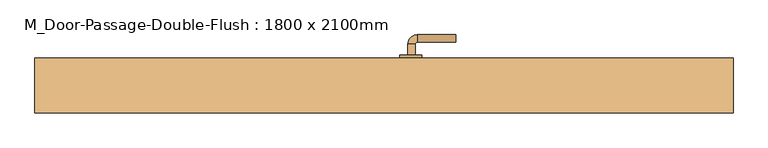
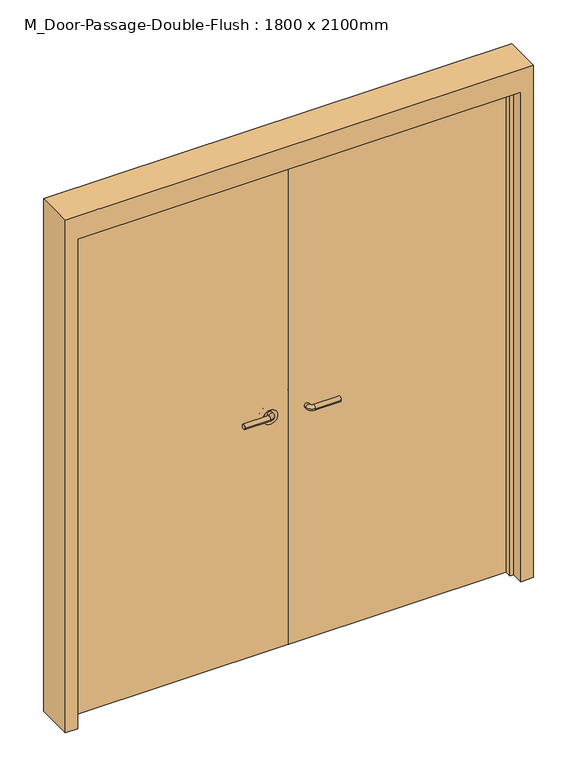
"""IFC4 building model written with IfcOpenShell, lengths in millimetres: door geometry, M_Door-Passage-Double-Flush : 1800 x 2100mm."""

import ifcopenshell
import ifcopenshell.guid

model = None  # the IFC model being written
_history = None  # IfcOwnerHistory: only IFC2X3 demands one
_inside = {}  # id of a spatial element -> (the spatial element, [elements in it])
_under = {}  # id of a project, library or spatial element -> (it, [spatial elements below it])
_declared = {}  # id of a project -> (the project, [libraries it declares])
_typed = {}  # id of a type object -> (the type object, [elements of that type])
_made_of = {}  # id of a material, layer set ... -> (it, [elements and type objects made of it])


def new_model(schema):
    """Start an empty IFC model of exactly this schema.

    Asked for "IFC4X3", IfcOpenShell would pick the latest addendum, in which some entities
    have other attributes; the version numbers below select the first issue.
    IFC2X3 requires an IfcOwnerHistory on every rooted entity: one is made here for all.
    """
    global model, _history
    if schema == "IFC4X3":
        model = ifcopenshell.file(schema_version=(4, 3, 0, 0))
    else:
        model = ifcopenshell.file(schema=schema)
    _inside.clear()
    _under.clear()
    _declared.clear()
    _typed.clear()
    _made_of.clear()
    _history = None
    if model.schema == "IFC2X3":
        org = make("IfcOrganization", Name="unknown")
        user = make(
            "IfcPersonAndOrganization",
            ThePerson=make("IfcPerson", FamilyName="unknown"),
            TheOrganization=org,
        )
        app = make(
            "IfcApplication",
            ApplicationDeveloper=org,
            Version="unknown",
            ApplicationFullName="unknown",
            ApplicationIdentifier="unknown",
        )
        _history = make(
            "IfcOwnerHistory",
            OwningUser=user,
            OwningApplication=app,
            ChangeAction="ADDED",
            CreationDate=0,
        )
    return model


def make(cls, **values):
    """One entity of the class cls with the attributes given. An attribute that is None is left unset."""
    return model.create_entity(
        cls, **{name: value for name, value in values.items() if value is not None}
    )


def rooted(cls, **values):
    """An entity with a GlobalId (a new one), such as an element, a storey or a relation."""
    return make(cls, GlobalId=ifcopenshell.guid.new(), OwnerHistory=_history, **values)


def si_unit(unit_type, name, prefix=None):
    """IfcSIUnit, for example si_unit("LENGTHUNIT", "METRE", prefix="MILLI")."""
    return make("IfcSIUnit", UnitType=unit_type, Prefix=prefix, Name=name)


def assignment(units):
    """IfcUnitAssignment: the units of a project."""
    return None if units is None else make("IfcUnitAssignment", Units=units)


def point(xyz):
    """IfcCartesianPoint."""
    return None if xyz is None else make("IfcCartesianPoint", Coordinates=xyz)


def direction(xyz):
    """IfcDirection."""
    return None if xyz is None else make("IfcDirection", DirectionRatios=xyz)


def frame(location, z_axis=None, x_axis=None):
    """IfcAxis2Placement3D, a coordinate frame: its origin and axes. An axis left out is left unset."""
    return make(
        "IfcAxis2Placement3D",
        Location=point(location),
        Axis=direction(z_axis),
        RefDirection=direction(x_axis),
    )


def frame_2d(location, x_axis=None):
    """IfcAxis2Placement2D, a coordinate frame in the plane: its origin and x axis."""
    return make(
        "IfcAxis2Placement2D", Location=point(location), RefDirection=direction(x_axis)
    )


def origin():
    """The frame at (0, 0, 0) with its axes left unset."""
    return frame((0.0, 0.0, 0.0))


def origin_with_axes():
    """The frame at (0, 0, 0) with the z axis (0, 0, 1) and the x axis (1, 0, 0) written out."""
    return frame((0.0, 0.0, 0.0), z_axis=(0.0, 0.0, 1.0), x_axis=(1.0, 0.0, 0.0))


def place(relative_to, where):
    """IfcLocalPlacement: puts the frame where relative to a parent placement (None: the world)."""
    return make(
        "IfcLocalPlacement", PlacementRelTo=relative_to, RelativePlacement=where
    )


def context(
    kind, dimensions, precision=None, world=None, true_north=None, identifier=None
):
    """IfcGeometricRepresentationContext, for example the 3D "Model" context."""
    return make(
        "IfcGeometricRepresentationContext",
        ContextIdentifier=identifier,
        ContextType=kind,
        CoordinateSpaceDimension=dimensions,
        Precision=precision,
        WorldCoordinateSystem=world,
        TrueNorth=true_north,
    )


def project(units=None, contexts=None):
    """IfcProject with its units and contexts."""
    return rooted(
        "IfcProject",
        Name="project",
        RepresentationContexts=contexts,
        UnitsInContext=assignment(units),
    )


def spatial(cls, under=None, at=None, **own):
    """A site, building, storey or space (cls), placed at a placement, below another one or the project."""
    s = rooted(cls, ObjectPlacement=at, **own)
    if under is not None:
        _under.setdefault(under.id(), (under, []))[1].append(s)
    return s


def polyline(points):
    """IfcPolyline through the points."""
    return make("IfcPolyline", Points=[point(p) for p in points])


def circle_curve(where, radius):
    """IfcCircle in the frame where."""
    return make("IfcCircle", Position=where, Radius=radius)


def ellipse_curve(where, semi_axis1, semi_axis2):
    """IfcEllipse in the frame where."""
    return make(
        "IfcEllipse", Position=where, SemiAxis1=semi_axis1, SemiAxis2=semi_axis2
    )


def trimmed(basis, trim1, trim2, sense, master):
    """IfcTrimmedCurve: the piece of a basis curve between two trims."""
    return make(
        "IfcTrimmedCurve",
        BasisCurve=basis,
        Trim1=trim1,
        Trim2=trim2,
        SenseAgreement=sense,
        MasterRepresentation=master,
    )


def segment(curve, same_sense, transition):
    """IfcCompositeCurveSegment."""
    return make(
        "IfcCompositeCurveSegment",
        Transition=transition,
        SameSense=same_sense,
        ParentCurve=curve,
    )


def composite_curve(segments, self_intersect=None):
    """IfcCompositeCurve: segments joined end to end."""
    return make("IfcCompositeCurve", Segments=segments, SelfIntersect=self_intersect)


def outline(outer, holes=None, kind="AREA"):
    """IfcArbitraryClosedProfileDef: a profile drawn as a closed curve; with holes, ...WithVoids."""
    if holes is None:
        return make("IfcArbitraryClosedProfileDef", ProfileType=kind, OuterCurve=outer)
    return make(
        "IfcArbitraryProfileDefWithVoids",
        ProfileType=kind,
        OuterCurve=outer,
        InnerCurves=holes,
    )


def extrude(swept, where, along, depth):
    """IfcExtrudedAreaSolid: the profile swept, set in the frame where, extruded along a direction by depth."""
    return make(
        "IfcExtrudedAreaSolid",
        SweptArea=swept,
        Position=where,
        ExtrudedDirection=direction(along),
        Depth=depth,
    )


def faces_of(points, faces, orient=None, outer=None):
    """IfcFace entities. A face is a list of loops; a loop is a list of indices into points, from 0.

    orient and outer hold one flag for each loop. By default every Orientation is true, the
    first loop of a face is its IfcFaceOuterBound and the others are IfcFaceBound.
    """
    made = []
    for i, loops in enumerate(faces):
        bounds = []
        for j, loop in enumerate(loops):
            is_outer = j == 0 if outer is None else outer[i][j]
            bounds.append(
                make(
                    "IfcFaceOuterBound" if is_outer else "IfcFaceBound",
                    Bound=make("IfcPolyLoop", Polygon=[points[k] for k in loop]),
                    Orientation=True if orient is None else orient[i][j],
                )
            )
        made.append(make("IfcFace", Bounds=bounds))
    return made


def faceted_brep(points, faces, orient=None, outer=None, voids=None):
    """IfcFacetedBrep: a solid bounded by flat faces; with voids (closed shells), ...WithVoids."""
    shared = [point(p) for p in points]
    hull = make("IfcClosedShell", CfsFaces=faces_of(shared, faces, orient, outer))
    if voids is None:
        return make("IfcFacetedBrep", Outer=hull)
    return make(
        "IfcFacetedBrepWithVoids",
        Outer=hull,
        Voids=[
            make(cls, CfsFaces=faces_of(shared, fs, o, b)) for cls, fs, o, b in voids
        ],
    )


def shape(context_of_items, identifier, shape_type, items):
    """IfcShapeRepresentation: the items that make up one representation, for example the "Body"."""
    return make(
        "IfcShapeRepresentation",
        ContextOfItems=context_of_items,
        RepresentationIdentifier=identifier,
        RepresentationType=shape_type,
        Items=items,
    )


def source(mapping_origin, context_of_items, identifier, shape_type, items):
    """IfcRepresentationMap: a shape defined once, which mapped items show again and again."""
    return make(
        "IfcRepresentationMap",
        MappingOrigin=mapping_origin,
        MappedRepresentation=shape(context_of_items, identifier, shape_type, items),
    )


def transform(
    local_origin,
    x_axis=None,
    y_axis=None,
    z_axis=None,
    scale=None,
    scale2=None,
    scale3=None,
    uniform=True,
):
    """IfcCartesianTransformationOperator3D, or its non-uniform kind. x_axis, y_axis, z_axis: its Axis1, 2, 3."""
    if uniform:
        return make(
            "IfcCartesianTransformationOperator3D",
            Axis1=direction(x_axis),
            Axis2=direction(y_axis),
            LocalOrigin=point(local_origin),
            Scale=scale,
            Axis3=direction(z_axis),
        )
    return make(
        "IfcCartesianTransformationOperator3DnonUniform",
        Axis1=direction(x_axis),
        Axis2=direction(y_axis),
        LocalOrigin=point(local_origin),
        Scale=scale,
        Axis3=direction(z_axis),
        Scale2=scale2,
        Scale3=scale3,
    )


def mapped(mapping_source, mapping_target):
    """IfcMappedItem: shows the shape of a source again, moved by a transform."""
    return make(
        "IfcMappedItem", MappingSource=mapping_source, MappingTarget=mapping_target
    )


def made_of(thing, what):
    """Note that an element or type object is made of a material, layer set ...; save() writes the relation."""
    if what is not None:
        _made_of.setdefault(what.id(), (what, []))[1].append(thing)
    return thing


def element(
    cls,
    number,
    at=None,
    inside=None,
    cuts=None,
    type_object=None,
    material=None,
    context=None,
    identifier="Body",
    shape_type=None,
    held_by="IfcProductDefinitionShape",
    body=None,
    shapes=None,
    **own,
):
    """One element of the class cls, such as IfcWall. Its Tag is "e" and its number.

    at: its placement. inside: the storey or other place that contains it. cuts: it is an
    opening in that element (IfcRelVoidsElement). A single representation is given by context,
    identifier, shape_type and body (its items); several are given by shapes. held_by: the class
    of the entity that holds the representations. save() writes the other relations.
    """
    e = rooted(cls, Tag="e%d" % number, ObjectPlacement=at, **own)
    if body is not None:
        shapes = [shape(context, identifier, shape_type, body)]
    if shapes is not None:
        e.Representation = make(held_by, Representations=shapes)
    if inside is not None:
        _inside.setdefault(inside.id(), (inside, []))[1].append(e)
    if cuts is not None:
        rooted(
            "IfcRelVoidsElement", RelatingBuildingElement=cuts, RelatedOpeningElement=e
        )
    if type_object is not None:
        _typed.setdefault(type_object.id(), (type_object, []))[1].append(e)
    return made_of(e, material)


def aggregate(whole, parts):
    """IfcRelAggregates: a whole, such as a stair, and the parts it consists of."""
    return rooted("IfcRelAggregates", RelatingObject=whole, RelatedObjects=parts)


def save(model, path):
    """Write the relations noted so far, then the file.

    IfcRelAggregates (storeys below a building ...), IfcRelContainedInSpatialStructure (elements
    in a storey), IfcRelDefinesByType, IfcRelAssociatesMaterial and IfcRelDeclares: one each for
    every whole, place, type object, material and project.
    """
    for whole, parts in _under.values():
        aggregate(whole, parts)
    for where, things in _inside.values():
        rooted(
            "IfcRelContainedInSpatialStructure",
            RelatedElements=things,
            RelatingStructure=where,
        )
    for kind, things in _typed.values():
        rooted("IfcRelDefinesByType", RelatedObjects=things, RelatingType=kind)
    for what, things in _made_of.values():
        rooted("IfcRelAssociatesMaterial", RelatedObjects=things, RelatingMaterial=what)
    for by, libraries in _declared.values():
        rooted("IfcRelDeclares", RelatingContext=by, RelatedDefinitions=libraries)
    model.write(path)


def plane_surface(at):
    """IfcPlane: the flat surface through the origin of the frame at, square to its z axis."""
    return make("IfcPlane", Position=at)


def cylinder_surface(at, radius):
    """IfcCylindricalSurface: all points at the distance radius from the z axis of the frame at."""
    return make("IfcCylindricalSurface", Position=at, Radius=radius)


def revolved_surface(curve, axis_point, axis_direction):
    """IfcSurfaceOfRevolution: the curve turned about the line through axis_point along axis_direction."""
    return make(
        "IfcSurfaceOfRevolution",
        SweptCurve=make("IfcArbitraryOpenProfileDef", ProfileType="CURVE", Curve=curve),
        AxisPosition=make("IfcAxis1Placement", Location=point(axis_point), Axis=direction(axis_direction)),
    )


def advanced_brep(points, edges, surfaces, faces):
    """IfcAdvancedBrep: a solid bounded by faces that lie on surfaces and meet in shared edges.

    An edge is (start, end): straight between two places in points (the first is 0);
    or (start, end, curve); or (start, end, curve, False) where it runs against its curve.
    A face is (place in surfaces, loops), or (place, loops, False) where it looks against
    its surface's normal. A loop lists edges by number (the first is 1), with a minus sign
    where the edge is run from its end to its start. The first loop is the outer one.
    """
    corners = [point(p) for p in points]
    vertices = [make("IfcVertexPoint", VertexGeometry=c) for c in corners]
    made = []
    for start, end, *more in edges:
        made.append(
            make(
                "IfcEdgeCurve",
                EdgeStart=vertices[start],
                EdgeEnd=vertices[end],
                EdgeGeometry=more[0] if more else make("IfcPolyline", Points=[corners[start], corners[end]]),
                SameSense=more[1] if len(more) > 1 else True,
            )
        )
    hull = []
    for where, loops, *sense in faces:
        bounds = []
        for j, loop in enumerate(loops):
            ring = [make("IfcOrientedEdge", EdgeElement=made[abs(k) - 1], Orientation=k > 0) for k in loop]
            bounds.append(
                make(
                    "IfcFaceOuterBound" if j == 0 else "IfcFaceBound",
                    Bound=make("IfcEdgeLoop", EdgeList=ring),
                    Orientation=True,
                )
            )
        hull.append(make("IfcAdvancedFace", Bounds=bounds, FaceSurface=surfaces[where], SameSense=sense[0] if sense else True))
    return make("IfcAdvancedBrep", Outer=make("IfcClosedShell", CfsFaces=hull))


def m_door_passage_double_flush_1800_x_2100mm_17443fe2(model_context):
    return source(origin(), model_context, "Body", "SolidModel", [
        advanced_brep(
        [(-65.009375, 102.85, 1016.0), (-85.009375, 102.85, 1016.0), (-65.009375, 72.85, 1016.0), (-85.009375, 72.85, 1016.0), (-90.009375, 67.85, 1016.0), (-90.009375, 47.85, 1016.0), (-195.009375, 47.85, 1016.0), (-195.009375, 67.85, 1016.0)],
        [
            (0, 1, circle_curve(frame((-75.009375, 102.85, 1016.0), z_axis=(0.0, 1.0, 0.0), x_axis=(-1.0, 0.0, 0.0)), 10.0)),
            (1, 0, circle_curve(frame((-75.009375, 102.85, 1016.0), z_axis=(0.0, 1.0, 0.0), x_axis=(-1.0, 0.0, 0.0)), 10.0)),
            (0, 2),
            (2, 3, circle_curve(frame((-75.009375, 72.85, 1016.0), z_axis=(0.0, 1.0, 0.0), x_axis=(-1.0, 0.0, 0.0)), 10.0)),
            (3, 1),
            (3, 2, circle_curve(frame((-75.009375, 72.85, 1016.0), z_axis=(0.0, 1.0, 0.0), x_axis=(-1.0, 0.0, 0.0)), 10.0)),
            (4, 3, circle_curve(frame((-90.009375, 72.85, 1016.0), z_axis=(0.0, 0.0, 1.0), x_axis=(1.0, 0.0, 0.0)), 5.0)),
            (2, 5, circle_curve(frame((-90.009375, 72.85, 1016.0), z_axis=(0.0, 0.0, -1.0), x_axis=(1.0, 0.0, 0.0)), 25.0)),
            (5, 4, circle_curve(frame((-90.009375, 57.85, 1016.0), z_axis=(1.0, 0.0, 0.0), x_axis=(0.0, 1.0, 0.0)), 10.0)),
            (4, 5, circle_curve(frame((-90.009375, 57.85, 1016.0), z_axis=(1.0, 0.0, 0.0), x_axis=(0.0, 1.0, 0.0)), 10.0)),
            (6, 7, circle_curve(frame((-195.009375, 57.85, 1016.0), z_axis=(-1.0, 0.0, 0.0), x_axis=(0.0, 1.0, 0.0)), 10.0)),
            (7, 6, circle_curve(frame((-195.009375, 57.85, 1016.0), z_axis=(-1.0, 0.0, 0.0), x_axis=(0.0, 1.0, 0.0)), 10.0)),
            (5, 6),
            (7, 4),
        ],
        [
            plane_surface(frame((-75.009375, 102.85, 1016.0), z_axis=(0.0, 1.0, 0.0), x_axis=(0.0, 0.0, 1.0))),
            cylinder_surface(frame((-75.009375, 102.85, 1016.0), z_axis=(0.0, 1.0, 0.0), x_axis=(-1.0, 0.0, 0.0)), 10.0),
            revolved_surface(trimmed(ellipse_curve(frame((-75.009375, 72.85, 1016.0), z_axis=(0.0, 1.0, 0.0), x_axis=(-1.0, 0.0, 0.0)), 10.0, 10.0), [point((-65.009375, 72.85, 1016.0))], [point((-85.009375, 72.85, 1016.0))], True, "CARTESIAN"), (-90.009375, 72.85, 1016.0), (0.0, 0.0, -1.0)),
            revolved_surface(trimmed(ellipse_curve(frame((-75.009375, 72.85, 1016.0), z_axis=(0.0, 1.0, 0.0), x_axis=(-1.0, 0.0, 0.0)), 10.0, 10.0), [point((-85.009375, 72.85, 1016.0))], [point((-65.009375, 72.85, 1016.0))], True, "CARTESIAN"), (-90.009375, 72.85, 1016.0), (0.0, 0.0, -1.0)),
            plane_surface(frame((-195.009375, 57.85, 1016.0), z_axis=(-1.0, 0.0, 0.0), x_axis=(0.0, 0.0, 1.0))),
            cylinder_surface(frame((-90.009375, 57.85, 1016.0), z_axis=(1.0, 0.0, 0.0), x_axis=(0.0, 1.0, 0.0)), 10.0),
        ],
        [
            (0, [[1, 2]]),
            (1, [[-1, 3, 4, 5]]),
            (1, [[-2, -5, 6, -3]]),
            (2, [[7, -4, 8, 9]]),
            (3, [[-8, -6, -7, 10]]),
            (4, [[11, 12]]),
            (5, [[-9, 13, -12, 14]]),
            (5, [[-10, -14, -11, -13]]),
        ],
    ),
        extrude(outline(composite_curve([segment(trimmed(circle_curve(frame_2d((1016.0, -72.509375)), 30.0), [point((1016.0, -42.509375))], [point((1016.0, -102.509375))], False, "CARTESIAN"), True, "CONTINUOUS"), segment(trimmed(circle_curve(frame_2d((1016.0, -72.509375)), 30.0), [point((1016.0, -102.509375))], [point((1016.0, -42.509375))], False, "CARTESIAN"), True, "CONTINUOUS")], self_intersect=False)), frame((0.0, 102.85, 0.0), z_axis=(0.0, 1.0, 0.0), x_axis=(0.0, 0.0, 1.0)), (0.0, 0.0, 1.0), 8.0),
        advanced_brep(
        [(-65.009375, 90.95, 1000.0), (-85.009375, 90.95, 1000.0), (-85.009375, 120.95, 1000.0), (-65.009375, 120.95, 1000.0), (-90.009375, 125.95, 1000.0), (-90.009375, 145.95, 1000.0), (-195.009375, 145.95, 1000.0), (-195.009375, 125.95, 1000.0)],
        [
            (0, 1, circle_curve(frame((-75.009375, 90.95, 1000.0), z_axis=(0.0, -1.0, 0.0), x_axis=(-1.0, 0.0, 0.0)), 10.0)),
            (1, 0, circle_curve(frame((-75.009375, 90.95, 1000.0), z_axis=(0.0, -1.0, 0.0), x_axis=(-1.0, 0.0, 0.0)), 10.0)),
            (1, 2),
            (2, 3, circle_curve(frame((-75.009375, 120.95, 1000.0), z_axis=(0.0, -1.0, 0.0), x_axis=(-1.0, 0.0, 0.0)), 10.0)),
            (3, 0),
            (3, 2, circle_curve(frame((-75.009375, 120.95, 1000.0), z_axis=(0.0, -1.0, 0.0), x_axis=(-1.0, 0.0, 0.0)), 10.0)),
            (4, 5, circle_curve(frame((-90.009375, 135.95, 1000.0), z_axis=(1.0, 0.0, 0.0), x_axis=(0.0, -1.0, 0.0)), 10.0)),
            (5, 3, circle_curve(frame((-90.009375, 120.95, 1000.0), z_axis=(0.0, 0.0, -1.0), x_axis=(1.0, 0.0, 0.0)), 25.0)),
            (2, 4, circle_curve(frame((-90.009375, 120.95, 1000.0), z_axis=(0.0, 0.0, 1.0), x_axis=(1.0, 0.0, 0.0)), 5.0)),
            (5, 4, circle_curve(frame((-90.009375, 135.95, 1000.0), z_axis=(1.0, 0.0, 0.0), x_axis=(0.0, -1.0, 0.0)), 10.0)),
            (6, 7, circle_curve(frame((-195.009375, 135.95, 1000.0), z_axis=(-1.0, 0.0, 0.0), x_axis=(0.0, -1.0, 0.0)), 10.0)),
            (7, 6, circle_curve(frame((-195.009375, 135.95, 1000.0), z_axis=(-1.0, 0.0, 0.0), x_axis=(0.0, -1.0, 0.0)), 10.0)),
            (4, 7),
            (6, 5),
        ],
        [
            plane_surface(frame((-75.009375, 90.95, 1000.0), z_axis=(0.0, -1.0, 0.0), x_axis=(0.0, 0.0, 1.0))),
            cylinder_surface(frame((-75.009375, 90.95, 1000.0), z_axis=(0.0, -1.0, 0.0), x_axis=(-1.0, 0.0, 0.0)), 10.0),
            revolved_surface(trimmed(ellipse_curve(frame((-75.009375, 120.95, 1000.0), z_axis=(0.0, 1.0, 0.0), x_axis=(-1.0, 0.0, 0.0)), 10.0, 10.0), [point((-65.009375, 120.95, 1000.0))], [point((-85.009375, 120.95, 1000.0))], True, "CARTESIAN"), (-90.009375, 120.95, 1000.0), (0.0, 0.0, -1.0)),
            revolved_surface(trimmed(ellipse_curve(frame((-75.009375, 120.95, 1000.0), z_axis=(0.0, 1.0, 0.0), x_axis=(-1.0, 0.0, 0.0)), 10.0, 10.0), [point((-85.009375, 120.95, 1000.0))], [point((-65.009375, 120.95, 1000.0))], True, "CARTESIAN"), (-90.009375, 120.95, 1000.0), (0.0, 0.0, -1.0)),
            plane_surface(frame((-195.009375, 135.95, 1000.0), z_axis=(-1.0, 0.0, 0.0), x_axis=(0.0, 0.0, 1.0))),
            cylinder_surface(frame((-90.009375, 135.95, 1000.0), z_axis=(1.0, 0.0, 0.0), x_axis=(0.0, -1.0, 0.0)), 10.0),
        ],
        [
            (0, [[1, 2]]),
            (1, [[3, 4, 5, -2]]),
            (1, [[-5, 6, -3, -1]]),
            (2, [[7, 8, -4, 9]]),
            (3, [[10, -9, -6, -8]]),
            (4, [[11, 12]]),
            (5, [[13, -11, 14, -7]]),
            (5, [[-14, -12, -13, -10]]),
        ],
    ),
        extrude(outline(composite_curve([segment(trimmed(circle_curve(frame_2d((1000.0, -72.509375)), 30.0), [point((1000.0, -42.509375))], [point((1000.0, -102.509375))], False, "CARTESIAN"), True, "CONTINUOUS"), segment(trimmed(circle_curve(frame_2d((1000.0, -72.509375)), 30.0), [point((1000.0, -102.509375))], [point((1000.0, -42.509375))], False, "CARTESIAN"), True, "CONTINUOUS")], self_intersect=False)), frame((0.0, 82.95, 0.0), z_axis=(0.0, 1.0, 0.0), x_axis=(0.0, 0.0, 1.0)), (0.0, 0.0, 1.0), 8.0),
        advanced_brep(
        [(65.009375, 102.85, 1000.0), (85.009375, 102.85, 1000.0), (85.009375, 72.85, 1000.0), (65.009375, 72.85, 1000.0), (90.009375, 67.85, 1000.0), (90.009375, 47.85, 1000.0), (195.009375, 47.85, 1000.0), (195.009375, 67.85, 1000.0)],
        [
            (0, 1, circle_curve(frame((75.009375, 102.85, 1000.0), z_axis=(0.0, 1.0, 0.0), x_axis=(1.0, 0.0, 0.0)), 10.0)),
            (1, 0, circle_curve(frame((75.009375, 102.85, 1000.0), z_axis=(0.0, 1.0, 0.0), x_axis=(1.0, 0.0, 0.0)), 10.0)),
            (1, 2),
            (2, 3, circle_curve(frame((75.009375, 72.85, 1000.0), z_axis=(0.0, 1.0, 0.0), x_axis=(1.0, 0.0, 0.0)), 10.0)),
            (3, 0),
            (3, 2, circle_curve(frame((75.009375, 72.85, 1000.0), z_axis=(0.0, 1.0, 0.0), x_axis=(1.0, 0.0, 0.0)), 10.0)),
            (4, 5, circle_curve(frame((90.009375, 57.85, 1000.0), z_axis=(-1.0, 0.0, 0.0), x_axis=(0.0, 1.0, 0.0)), 10.0)),
            (5, 3, circle_curve(frame((90.009375, 72.85, 1000.0), z_axis=(0.0, 0.0, -1.0), x_axis=(-1.0, 0.0, 0.0)), 25.0)),
            (2, 4, circle_curve(frame((90.009375, 72.85, 1000.0), z_axis=(0.0, 0.0, 1.0), x_axis=(-1.0, 0.0, 0.0)), 5.0)),
            (5, 4, circle_curve(frame((90.009375, 57.85, 1000.0), z_axis=(-1.0, 0.0, 0.0), x_axis=(0.0, 1.0, 0.0)), 10.0)),
            (6, 7, circle_curve(frame((195.009375, 57.85, 1000.0), z_axis=(1.0, 0.0, 0.0), x_axis=(0.0, 1.0, 0.0)), 10.0)),
            (7, 6, circle_curve(frame((195.009375, 57.85, 1000.0), z_axis=(1.0, 0.0, 0.0), x_axis=(0.0, 1.0, 0.0)), 10.0)),
            (4, 7),
            (6, 5),
        ],
        [
            plane_surface(frame((75.009375, 102.85, 1000.0), z_axis=(0.0, 1.0, 0.0), x_axis=(0.0, 0.0, 1.0))),
            cylinder_surface(frame((75.009375, 102.85, 1000.0), z_axis=(0.0, 1.0, 0.0), x_axis=(1.0, 0.0, 0.0)), 10.0),
            revolved_surface(trimmed(ellipse_curve(frame((75.009375, 72.85, 1000.0), z_axis=(0.0, -1.0, 0.0), x_axis=(1.0, 0.0, 0.0)), 10.0, 10.0), [point((65.009375, 72.85, 1000.0))], [point((85.009375, 72.85, 1000.0))], True, "CARTESIAN"), (90.009375, 72.85, 1000.0), (0.0, 0.0, -1.0)),
            revolved_surface(trimmed(ellipse_curve(frame((75.009375, 72.85, 1000.0), z_axis=(0.0, -1.0, 0.0), x_axis=(1.0, 0.0, 0.0)), 10.0, 10.0), [point((85.009375, 72.85, 1000.0))], [point((65.009375, 72.85, 1000.0))], True, "CARTESIAN"), (90.009375, 72.85, 1000.0), (0.0, 0.0, -1.0)),
            plane_surface(frame((195.009375, 57.85, 1000.0), z_axis=(1.0, 0.0, 0.0), x_axis=(0.0, 0.0, 1.0))),
            cylinder_surface(frame((90.009375, 57.85, 1000.0), z_axis=(-1.0, 0.0, 0.0), x_axis=(0.0, 1.0, 0.0)), 10.0),
        ],
        [
            (0, [[1, 2]]),
            (1, [[3, 4, 5, -2]]),
            (1, [[-5, 6, -3, -1]]),
            (2, [[7, 8, -4, 9]]),
            (3, [[10, -9, -6, -8]]),
            (4, [[11, 12]]),
            (5, [[13, -11, 14, -7]]),
            (5, [[-14, -12, -13, -10]]),
        ],
    ),
        extrude(outline(composite_curve([segment(trimmed(circle_curve(frame_2d((1000.0, 72.509375)), 30.0), [point((1000.0, 42.509375))], [point((1000.0, 102.509375))], False, "CARTESIAN"), True, "CONTINUOUS"), segment(trimmed(circle_curve(frame_2d((1000.0, 72.509375)), 30.0), [point((1000.0, 102.509375))], [point((1000.0, 42.509375))], False, "CARTESIAN"), True, "CONTINUOUS")], self_intersect=False)), frame((0.0, 102.85, 0.0), z_axis=(0.0, 1.0, 0.0), x_axis=(0.0, 0.0, 1.0)), (0.0, 0.0, 1.0), 8.0),
        advanced_brep(
        [(65.009375, 163.85, 1000.0), (85.009375, 163.85, 1000.0), (65.009375, 193.85, 1000.0), (85.009375, 193.85, 1000.0), (90.009375, 198.85, 1000.0), (90.009375, 218.85, 1000.0), (195.009375, 218.85, 1000.0), (195.009375, 198.85, 1000.0)],
        [
            (0, 1, circle_curve(frame((75.009375, 163.85, 1000.0), z_axis=(0.0, -1.0, 0.0), x_axis=(1.0, 0.0, 0.0)), 10.0)),
            (1, 0, circle_curve(frame((75.009375, 163.85, 1000.0), z_axis=(0.0, -1.0, 0.0), x_axis=(1.0, 0.0, 0.0)), 10.0)),
            (0, 2),
            (2, 3, circle_curve(frame((75.009375, 193.85, 1000.0), z_axis=(0.0, -1.0, 0.0), x_axis=(1.0, 0.0, 0.0)), 10.0)),
            (3, 1),
            (3, 2, circle_curve(frame((75.009375, 193.85, 1000.0), z_axis=(0.0, -1.0, 0.0), x_axis=(1.0, 0.0, 0.0)), 10.0)),
            (4, 3, circle_curve(frame((90.009375, 193.85, 1000.0), z_axis=(0.0, 0.0, 1.0), x_axis=(-1.0, 0.0, 0.0)), 5.0)),
            (2, 5, circle_curve(frame((90.009375, 193.85, 1000.0), z_axis=(0.0, 0.0, -1.0), x_axis=(-1.0, 0.0, 0.0)), 25.0)),
            (5, 4, circle_curve(frame((90.009375, 208.85, 1000.0), z_axis=(-1.0, 0.0, 0.0), x_axis=(0.0, -1.0, 0.0)), 10.0)),
            (4, 5, circle_curve(frame((90.009375, 208.85, 1000.0), z_axis=(-1.0, 0.0, 0.0), x_axis=(0.0, -1.0, 0.0)), 10.0)),
            (6, 7, circle_curve(frame((195.009375, 208.85, 1000.0), z_axis=(1.0, 0.0, 0.0), x_axis=(0.0, -1.0, 0.0)), 10.0)),
            (7, 6, circle_curve(frame((195.009375, 208.85, 1000.0), z_axis=(1.0, 0.0, 0.0), x_axis=(0.0, -1.0, 0.0)), 10.0)),
            (5, 6),
            (7, 4),
        ],
        [
            plane_surface(frame((75.009375, 163.85, 1000.0), z_axis=(0.0, -1.0, 0.0), x_axis=(0.0, 0.0, 1.0))),
            cylinder_surface(frame((75.009375, 163.85, 1000.0), z_axis=(0.0, -1.0, 0.0), x_axis=(1.0, 0.0, 0.0)), 10.0),
            revolved_surface(trimmed(ellipse_curve(frame((75.009375, 193.85, 1000.0), z_axis=(0.0, -1.0, 0.0), x_axis=(1.0, 0.0, 0.0)), 10.0, 10.0), [point((65.009375, 193.85, 1000.0))], [point((85.009375, 193.85, 1000.0))], True, "CARTESIAN"), (90.009375, 193.85, 1000.0), (0.0, 0.0, -1.0)),
            revolved_surface(trimmed(ellipse_curve(frame((75.009375, 193.85, 1000.0), z_axis=(0.0, -1.0, 0.0), x_axis=(1.0, 0.0, 0.0)), 10.0, 10.0), [point((85.009375, 193.85, 1000.0))], [point((65.009375, 193.85, 1000.0))], True, "CARTESIAN"), (90.009375, 193.85, 1000.0), (0.0, 0.0, -1.0)),
            plane_surface(frame((195.009375, 208.85, 1000.0), z_axis=(1.0, 0.0, 0.0), x_axis=(0.0, 0.0, 1.0))),
            cylinder_surface(frame((90.009375, 208.85, 1000.0), z_axis=(-1.0, 0.0, 0.0), x_axis=(0.0, -1.0, 0.0)), 10.0),
        ],
        [
            (0, [[1, 2]]),
            (1, [[-1, 3, 4, 5]]),
            (1, [[-2, -5, 6, -3]]),
            (2, [[7, -4, 8, 9]]),
            (3, [[-8, -6, -7, 10]]),
            (4, [[11, 12]]),
            (5, [[-9, 13, -12, 14]]),
            (5, [[-10, -14, -11, -13]]),
        ],
    ),
        extrude(outline(composite_curve([segment(trimmed(circle_curve(frame_2d((1000.0, 72.509375)), 30.0), [point((1000.0, 42.509375))], [point((1000.0, 102.509375))], False, "CARTESIAN"), True, "CONTINUOUS"), segment(trimmed(circle_curve(frame_2d((1000.0, 72.509375)), 30.0), [point((1000.0, 102.509375))], [point((1000.0, 42.509375))], False, "CARTESIAN"), True, "CONTINUOUS")], self_intersect=False)), frame((0.0, 155.85, 0.0), z_axis=(0.0, 1.0, 0.0), x_axis=(0.0, 0.0, 1.0)), (0.0, 0.0, 1.0), 8.0),
        extrude(outline(polyline([(900.0, 82.95), (1.5875, 82.95), (1.5875, 110.85), (900.0, 110.85), (900.0, 82.95)])), origin_with_axes(), (0.0, 0.0, 1.0), 2100.0),
        extrude(outline(polyline([(-1.5875, 82.95), (-900.0, 82.95), (-900.0, 110.85), (-1.5875, 110.85), (-1.5875, 82.95)])), origin_with_axes(), (0.0, 0.0, 1.0), 2100.0),
        faceted_brep([(900.0, 106.0875, 0.0), (900.0, 155.85, 0.0), (950.0, 155.85, 0.0), (950.0, 5.85, 0.0), (900.0, 5.85, 0.0), (900.0, 55.0625, 0.0), (884.125, 55.0625, 0.0), (884.125, 106.0875, 0.0), (900.0, 106.0875, 2100.0), (900.0, 155.85, 2100.0), (-900.0, 155.85, 2100.0), (-900.0, 155.85, 0.0), (-950.0, 155.85, 0.0), (-950.0, 155.85, 2200.0), (950.0, 155.85, 2200.0), (950.0, 5.85, 2200.0), (-950.0, 5.85, 2200.0), (-950.0, 5.85, 0.0), (-900.0, 5.85, 0.0), (-900.0, 5.85, 2100.0), (900.0, 5.85, 2100.0), (900.0, 55.0625, 2100.0), (-900.0, 55.0625, 2100.0), (-900.0, 55.0625, 0.0), (-884.125, 55.0625, 0.0), (-884.125, 55.0625, 2084.125), (884.125, 55.0625, 2084.125), (884.125, 106.0875, 2084.125), (-884.125, 106.0875, 2084.125), (-884.125, 106.0875, 0.0), (-900.0, 106.0875, 0.0), (-900.0, 106.0875, 2100.0)], [[[0, 1, 2, 3, 4, 5, 6, 7]], [[1, 0, 8, 9]], [[2, 1, 9, 10, 11, 12, 13, 14]], [[3, 2, 14, 15]], [[4, 3, 15, 16, 17, 18, 19, 20]], [[5, 4, 20, 21]], [[6, 5, 21, 22, 23, 24, 25, 26]], [[7, 6, 26, 27]], [[0, 7, 27, 28, 29, 30, 31, 8]], [[9, 8, 31, 10]], [[20, 19, 22, 21]], [[26, 25, 28, 27]], [[12, 11, 30, 29, 24, 23, 18, 17]], [[11, 10, 31, 30]], [[13, 12, 17, 16]], [[19, 18, 23, 22]], [[25, 24, 29, 28]], [[15, 14, 13, 16]]]),
    ])


if __name__ == "__main__":
    model = new_model("IFC4")
    model_context = context("Model", 3, world=origin())
    ifc_project = project(units=[si_unit("LENGTHUNIT", "METRE", prefix="MILLI")], contexts=[model_context])
    site = spatial("IfcSite", under=ifc_project)
    building = spatial("IfcBuilding", under=site)
    placement = place(None, origin())
    m_door_passage_double_flush_1800_x_2100mm_shape = m_door_passage_double_flush_1800_x_2100mm_17443fe2(model_context)
    element("IfcDoor", 1, ObjectType="M_Door-Passage-Double-Flush : 1800 x 2100mm", at=placement, inside=building, context=model_context, shape_type="MappedRepresentation", body=[
        mapped(m_door_passage_double_flush_1800_x_2100mm_shape, transform((0.0, 0.0, 0.0), x_axis=(1.0, 0.0, 0.0), y_axis=(0.0, 1.0, 0.0), z_axis=(0.0, 0.0, 1.0))),
    ])
    save(model, "model.ifc")

# Revit data of these elements
# Type "M_Door-Passage-Double-Flush : 1800 x 2100mm"
#   Type Mark = "34"
#   Assembly Code = "B2030200"
#   Analytic Construction = "Metal"
#   Thickness = 45 mm
#   Thermal Resistance (R) = 0.270118 (m²·K)/W
#   Swing Angle [instance default] = 90.00°
#   Strike Height = 1000 mm
#   SinglePanelWidth = 900 mm
#   Rough Width [instance default] = 1900 mm
#   Rough Height [instance default] = 2200 mm
#   MFOpeningHeight [instance default] = 100 mm
#   MFOpeningWidth [instance default] = 100 mm
#   Inset Calculate [instance default] = 105 mm
#   Masonry Inset [instance default] = 25 mm
#   Height = 2100 mm
#   Width = 1800 mm
#   Heat Transfer Coefficient (U) = 3.70223 W/(m²·K)
#   Masonry Frame Depth = 150 mm
#   Masonry Frame [instance default] = yes
#   Function = 1
#   Dry Wall Frame [instance default] = no
#   Panel Material = Metal Door - Brindle
#   Frame Material = Metal - Painted - Grey
#   Door Handle Material = Aluminum
#   Visual Light Transmittance = 0
#   Solar Heat Gain Coefficient = 0
#   Wall Closure = (empty or 0)
# Element 1 (IfcDoor, "M_Door-Passage-Double-Flush : 1800 x 2100mm")
#   Materials on its faces: "Aluminum", "Metal - Painted - Grey", "Metal Door - Brindle"
# Materials
#   "Metal Door - Brindle": class "Paint", colour RGB 164 133 98, transparency 0
#   "Metal - Painted - Grey": class "Paint", colour RGB 104 104 104, transparency 0
#   "Aluminum": class "Metal", colour RGB 244 245 246, transparency 0, Description = "Aluminum 6061", Cost = 0
